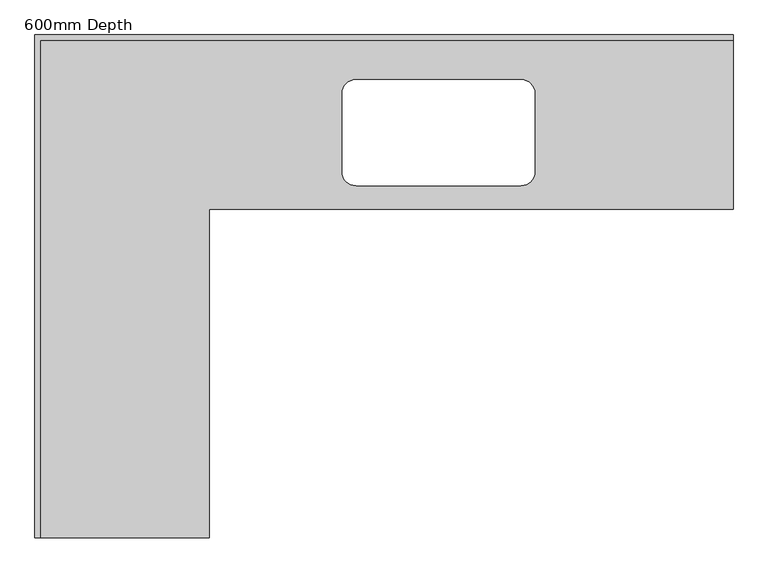
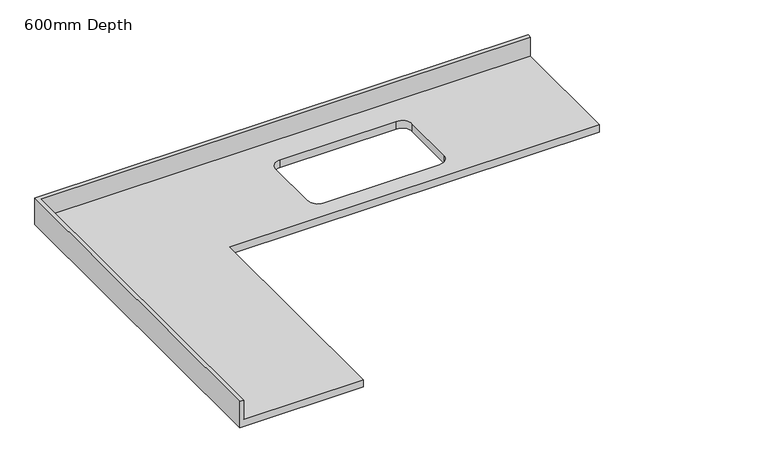
"""IFC4 building model written with IfcOpenShell, lengths in millimetres: furniture geometry, M_Counter Top-L Shaped w Sink : 600mm Depth."""

from ifc_helpers import new_model, si_unit, frame, origin, place, context, project, spatial, polyline, circle_curve, source, transform, mapped, element, save
from ifc_brep_helpers import plane_surface, revolved_surface, advanced_brep


def furniture_600mm_depth_33a330ac(model_context):
    return source(origin(), model_context, "Body", "AdvancedBrep", [
        advanced_brep(
        [(-575.4622951, -1800.0, 900.0), (-575.4622951, -625.0, 900.0), (1299.5377049, -625.0, 900.0), (1299.5377049, -19.05, 900.0), (-1181.4122951, -19.05, 900.0), (-1181.4122951, -1800.0, 900.0), (539.5377049, -160.0, 900.0), (589.5377049, -210.0, 900.0), (589.5377049, -490.0, 900.0), (539.5377049, -540.0, 900.0), (-50.4622951, -540.0, 900.0), (-100.4622951, -490.0, 900.0), (-100.4622951, -210.0, 900.0), (-50.4622951, -160.0, 900.0), (1299.5377049, 0.0, 860.0), (1299.5377049, -625.0, 860.0), (-575.4622951, -625.0, 860.0), (-575.4622951, -1800.0, 860.0), (-1200.4622951, -1800.0, 860.0), (-1200.4622951, 0.0, 860.0), (539.5377049, -160.0, 860.0), (-50.4622951, -160.0, 860.0), (-100.4622951, -210.0, 860.0), (-100.4622951, -490.0, 860.0), (-50.4622951, -540.0, 860.0), (539.5377049, -540.0, 860.0), (589.5377049, -490.0, 860.0), (589.5377049, -210.0, 860.0), (-1200.4622951, 0.0, 1001.6), (1299.5377049, 0.0, 1001.6), (-1200.4622951, -1800.0, 1001.6), (-1181.4122951, -1800.0, 1001.6), (1299.5377049, -19.05, 1001.6), (-1181.4122951, -19.05, 1001.6)],
        [
            (0, 1),
            (1, 2),
            (2, 3),
            (3, 4),
            (4, 5),
            (5, 0),
            (6, 7, circle_curve(frame((539.5377049, -210.0, 900.0), z_axis=(0.0, 0.0, -1.0), x_axis=(1.0, 0.0, 0.0)), 50.0)),
            (7, 8),
            (8, 9, circle_curve(frame((539.5377049, -490.0, 900.0), z_axis=(0.0, 0.0, -1.0), x_axis=(1.0, 0.0, 0.0)), 50.0)),
            (9, 10),
            (10, 11, circle_curve(frame((-50.4622951, -490.0, 900.0), z_axis=(0.0, 0.0, -1.0), x_axis=(1.0, 0.0, 0.0)), 50.0)),
            (11, 12),
            (12, 13, circle_curve(frame((-50.4622951, -210.0, 900.0), z_axis=(0.0, 0.0, -1.0), x_axis=(1.0, 0.0, 0.0)), 50.0)),
            (13, 6),
            (14, 15),
            (15, 16),
            (16, 17),
            (17, 18),
            (18, 19),
            (19, 14),
            (20, 21),
            (21, 22, circle_curve(frame((-50.4622951, -210.0, 860.0), z_axis=(0.0, 0.0, 1.0), x_axis=(1.0, 0.0, 0.0)), 50.0)),
            (22, 23),
            (23, 24, circle_curve(frame((-50.4622951, -490.0, 860.0), z_axis=(0.0, 0.0, 1.0), x_axis=(1.0, 0.0, 0.0)), 50.0)),
            (24, 25),
            (25, 26, circle_curve(frame((539.5377049, -490.0, 860.0), z_axis=(0.0, 0.0, 1.0), x_axis=(1.0, 0.0, 0.0)), 50.0)),
            (26, 27),
            (27, 20, circle_curve(frame((539.5377049, -210.0, 860.0), z_axis=(0.0, 0.0, 1.0), x_axis=(1.0, 0.0, 0.0)), 50.0)),
            (19, 28),
            (28, 29),
            (29, 14),
            (18, 30),
            (30, 28),
            (17, 0),
            (5, 31),
            (31, 30),
            (16, 1),
            (15, 2),
            (29, 32),
            (32, 3),
            (6, 20),
            (27, 7),
            (26, 8),
            (25, 9),
            (24, 10),
            (23, 11),
            (22, 12),
            (21, 13),
            (31, 33),
            (33, 32),
            (33, 4),
        ],
        [
            plane_surface(frame((-1200.4622951, 0.0, 900.0), z_axis=(0.0, 0.0, 1.0), x_axis=(-1.0, 0.0, 0.0))),
            plane_surface(frame((-1200.4622951, 0.0, 860.0), z_axis=(0.0, 0.0, -1.0), x_axis=(1.0, 0.0, 0.0))),
            plane_surface(frame((1299.5377049, 0.0, 900.0), z_axis=(0.0, 1.0, 0.0), x_axis=(0.0, 0.0, -1.0))),
            plane_surface(frame((-1200.4622951, 0.0, 900.0), z_axis=(-1.0, 0.0, 0.0), x_axis=(0.0, 0.0, -1.0))),
            plane_surface(frame((-1200.4622951, -1800.0, 900.0), z_axis=(0.0, -1.0, 0.0), x_axis=(0.0, 0.0, -1.0))),
            plane_surface(frame((-575.4622951, -1800.0, 900.0), z_axis=(1.0, 0.0, 0.0), x_axis=(0.0, 0.0, -1.0))),
            plane_surface(frame((-575.4622951, -625.0, 900.0), z_axis=(0.0, -1.0, 0.0), x_axis=(0.0, 0.0, -1.0))),
            plane_surface(frame((1299.5377049, -625.0, 900.0), z_axis=(1.0, 0.0, 0.0), x_axis=(0.0, 0.0, -1.0))),
            revolved_surface(polyline([(589.5377049, -210.0, 860.0), (589.5377049, -210.0, 900.0)]), (539.5377049, -210.0, 0.0), (0.0, 0.0, -1.0)),
            plane_surface(frame((589.5377049, -210.0, 900.0), z_axis=(-1.0, 0.0, 0.0), x_axis=(0.0, 0.0, -1.0))),
            revolved_surface(polyline([(589.5377049, -490.0, 860.0), (589.5377049, -490.0, 900.0)]), (539.5377049, -490.0, 0.0), (0.0, 0.0, -1.0)),
            plane_surface(frame((539.5377049, -540.0, 900.0), z_axis=(0.0, 1.0, 0.0), x_axis=(0.0, 0.0, -1.0))),
            revolved_surface(polyline([(-0.4622950999999986, -490.0, 860.0), (-0.4622950999999986, -490.0, 900.0)]), (-50.4622951, -490.0, 0.0), (0.0, 0.0, -1.0)),
            plane_surface(frame((-100.4622951, -490.0, 900.0), z_axis=(1.0, 0.0, 0.0), x_axis=(0.0, 0.0, -1.0))),
            revolved_surface(polyline([(-0.4622950999999986, -210.0, 860.0), (-0.4622950999999986, -210.0, 900.0)]), (-50.4622951, -210.0, 0.0), (0.0, 0.0, -1.0)),
            plane_surface(frame((-50.4622951, -160.0, 900.0), z_axis=(0.0, -1.0, 0.0), x_axis=(0.0, 0.0, -1.0))),
            plane_surface(frame((-1200.4622951, 0.0, 1001.6), z_axis=(0.0, 0.0, 1.0), x_axis=(0.0, -1.0, 0.0))),
            plane_surface(frame((-1200.4622951, -19.05, 1001.6), z_axis=(0.0, -1.0, 0.0), x_axis=(0.0, 0.0, -1.0))),
            plane_surface(frame((-1181.4122951, -1800.0, 1001.6), z_axis=(1.0, 0.0, 0.0), x_axis=(0.0, 0.0, -1.0))),
        ],
        [
            (0, [[1, 2, 3, 4, 5, 6], [7, 8, 9, 10, 11, 12, 13, 14]]),
            (1, [[15, 16, 17, 18, 19, 20], [21, 22, 23, 24, 25, 26, 27, 28]]),
            (2, [[-20, 29, 30, 31]]),
            (3, [[-19, 32, 33, -29]]),
            (4, [[-32, -18, 34, -6, 35, 36]]),
            (5, [[-1, -34, -17, 37]]),
            (6, [[-2, -37, -16, 38]]),
            (7, [[-15, -31, 39, 40, -3, -38]]),
            (8, [[-7, 41, -28, 42]]),
            (9, [[-8, -42, -27, 43]]),
            (10, [[-9, -43, -26, 44]]),
            (11, [[-10, -44, -25, 45]]),
            (12, [[-11, -45, -24, 46]]),
            (13, [[-12, -46, -23, 47]]),
            (14, [[-13, -47, -22, 48]]),
            (15, [[-14, -48, -21, -41]]),
            (16, [[-33, -36, 49, 50, -39, -30]]),
            (17, [[-40, -50, 51, -4]]),
            (18, [[-49, -35, -5, -51]]),
        ],
    ),
    ])


if __name__ == "__main__":
    model = new_model("IFC4")
    model_context = context("Model", 3, world=origin())
    ifc_project = project(units=[si_unit("LENGTHUNIT", "METRE", prefix="MILLI")], contexts=[model_context])
    site = spatial("IfcSite", under=ifc_project)
    building = spatial("IfcBuilding", under=site)
    placement = place(None, origin())
    furniture_600mm_depth_shape = furniture_600mm_depth_33a330ac(model_context)
    element("IfcFurniture", 1, ObjectType="M_Counter Top-L Shaped w Sink : 600mm Depth", at=placement, inside=building, context=model_context, shape_type="MappedRepresentation", body=[
        mapped(furniture_600mm_depth_shape, transform((0.0, 0.0, 0.0), x_axis=(1.0, 0.0, 0.0), y_axis=(0.0, 1.0, 0.0), z_axis=(0.0, 0.0, 1.0))),
    ])
    save(model, "model.ifc")

# Revit data of these elements
# Type "M_Counter Top-L Shaped w Sink : 600mm Depth"
#   Counter Thickness = 0.04 m
#   Depth = 0.625 m
#   Height = 0.90 m
#   Length - Leg 1 [instance default] = 2.50 m
#   Length - Leg 2 [instance default] = 1.80 m
#   Sink Location [instance default] = 1.10 m
#   Sink Location To Wall [instance default] = 0.16 m
#   Sink Opening Depth [instance default] = 0.38 m
#   Sink Opening Width [instance default] = 0.69 m
#   Counter Top Material = none
# Element 1 (IfcFurniture, "M_Counter Top-L Shaped w Sink : 600mm Depth")
#   Materials on its faces: "Counter Top"
# Materials
#   "Counter Top": class "Wood", colour RGB 226 177 128, transparency 0
